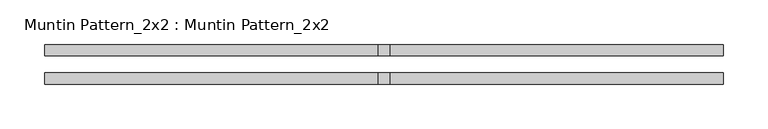
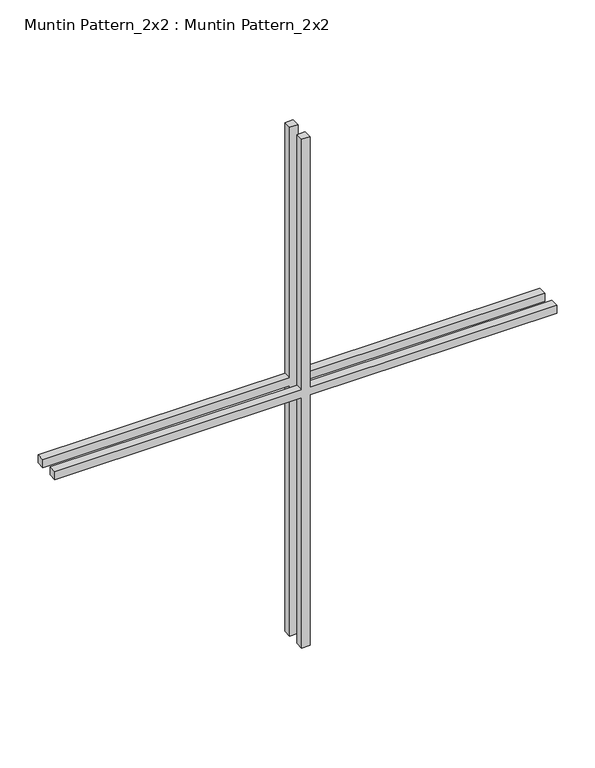
"""IFC4 building model written with IfcOpenShell, lengths in millimetres: proxy geometry, Muntin Pattern_2x2 : Muntin Pattern_2x2."""

from ifc_helpers import new_model, si_unit, frame, origin, place, context, project, spatial, polyline, outline, extrude, source, transform, mapped, element, save


def muntin_pattern_2x2_muntin_pattern_2x2_74d79337(model_context):
    return source(origin(), model_context, "Body", "SweptSolid", [
        extrude(outline(polyline([(414.3375, -6.35), (414.3375, -381.0), (401.6375, -381.0), (401.6375, -6.35), (0.0, -6.35), (0.0, 6.35), (401.6375, 6.35), (401.6375, 381.0), (414.3375, 381.0), (414.3375, 6.35), (815.975, 6.35), (815.975, -6.35), (414.3375, -6.35)])), frame((0.0, -22.225, 0.0), z_axis=(0.0, 1.0, 0.0), x_axis=(0.0, 0.0, 1.0)), (0.0, 0.0, 1.0), 12.7),
        extrude(outline(polyline([(414.3375, -6.35), (414.3375, -381.0), (401.6375, -381.0), (401.6375, -6.35), (0.0, -6.35), (0.0, 6.35), (401.6375, 6.35), (401.6375, 381.0), (414.3375, 381.0), (414.3375, 6.35), (815.975, 6.35), (815.975, -6.35), (414.3375, -6.35)])), frame((0.0, 9.525, 0.0), z_axis=(0.0, 1.0, 0.0), x_axis=(0.0, 0.0, 1.0)), (0.0, 0.0, 1.0), 12.7),
    ])


if __name__ == "__main__":
    model = new_model("IFC4")
    model_context = context("Model", 3, world=origin())
    ifc_project = project(units=[si_unit("LENGTHUNIT", "METRE", prefix="MILLI")], contexts=[model_context])
    site = spatial("IfcSite", under=ifc_project)
    building = spatial("IfcBuilding", under=site)
    placement = place(None, origin())
    muntin_pattern_2x2_muntin_pattern_2x2_shape = muntin_pattern_2x2_muntin_pattern_2x2_74d79337(model_context)
    element("IfcBuildingElementProxy", 1, Name="Muntin Pattern_2x2 : Muntin Pattern_2x2", ObjectType="Muntin Pattern_2x2 : Muntin Pattern_2x2", at=placement, inside=building, context=model_context, shape_type="MappedRepresentation", body=[
        mapped(muntin_pattern_2x2_muntin_pattern_2x2_shape, transform((0.0, 0.0, 0.0), x_axis=(1.0, 0.0, 0.0), y_axis=(0.0, 1.0, 0.0), z_axis=(0.0, 0.0, 1.0))),
    ])
    save(model, "model.ifc")

# Revit data of these elements
# Type "Muntin Pattern_2x2 : Muntin Pattern_2x2"
#   Width [instance default] = 4' - 0"
#   Thickness = 0' - 0 1/2"
#   Height [instance default] = 4' - 0"
#   Distance = 0' - 0 3/4"
#   Interior Material [instance default] = none
#   Exterior Material [instance default] = none
#   Default Elevation = 0
# Element 1 (IfcBuildingElementProxy, "Muntin Pattern_2x2 : Muntin Pattern_2x2")
#   Width = 2' - 6"
#   Height = 2' - 8 1/8"
#   Interior Material = Wood - Stained
#   Exterior Material = Clad - White
#   Materials on its faces: "Clad - White", "Wood - Stained"
# Materials
#   "Clad - White": class "Wood", colour RGB 242 242 238, transparency 0, Cost = 0
#   "Wood - Stained": class "Wood", colour RGB 224 178 126, transparency 0, Cost = 0
